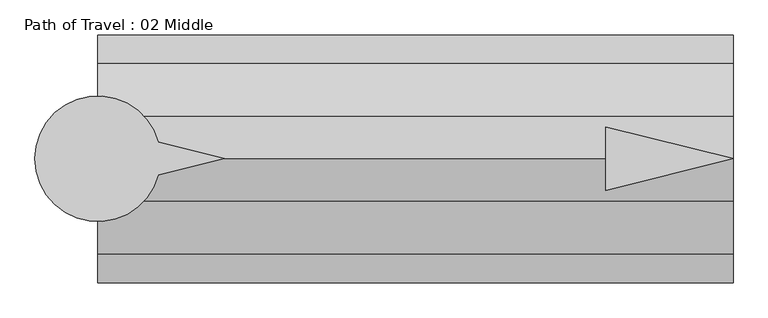
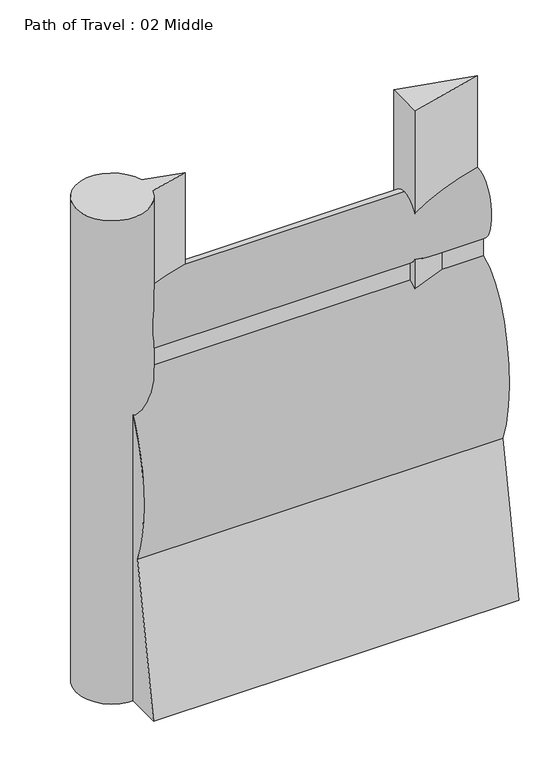
"""IFC4 building model written with IfcOpenShell, lengths in millimetres: proxy geometry, Path of Travel : 02 Middle."""

from ifc_helpers import new_model, si_unit, point, frame, frame_2d, origin, origin_with_axes, place, context, project, spatial, polyline, circle_curve, ellipse_curve, trimmed, segment, composite_curve, outline, extrude, source, transform, mapped, element, save
from ifc_brep_helpers import plane_surface, extruded_surface, advanced_brep


def path_of_travel_02_middle_987670bd(model_context):
    return source(origin(), model_context, "Body", "SolidModel", [
        advanced_brep(
        [(227.5554837, 0.0, 1727.2), (227.5554837, 42.9018657, 1436.6534209), (227.5554837, 42.9018657, 1363.4763406), (227.5554837, 184.1186263, 643.4144547), (227.5554837, 297.5699544, 0.0), (227.5554837, 145.6574193, 0.0), (227.5554837, 0.0, 584.2), (227.5554837, -145.6574193, 0.0), (227.5554837, -297.5699544, 0.0), (227.5554837, -184.1186263, 643.4144547), (227.5554837, -42.9018657, 1363.4763406), (227.5554837, -42.9018657, 1436.6534209), (1751.5554837, 0.0, 1727.2), (1751.5554837, -42.9018657, 1436.6534209), (1751.5554837, -42.9018657, 1363.4763406), (1751.5554837, -184.1186263, 643.4144547), (1751.5554837, -297.5699544, 0.0), (1751.5554837, -145.6574193, 0.0), (1751.5554837, 0.0, 584.2), (1751.5554837, 145.6574193, 0.0), (1751.5554837, 297.5699544, 0.0), (1751.5554837, 184.1186263, 643.4144547), (1751.5554837, 42.9018657, 1363.4763406), (1751.5554837, 42.9018657, 1436.6534209)],
        [
            (0, 1, ellipse_curve(frame((227.5554837, 0.0, 1574.8), z_axis=(-1.0, 0.0, 0.0), x_axis=(0.0, 0.0, 1.0)), 152.4, 101.6)),
            (1, 2),
            (2, 3, ellipse_curve(frame((227.5554837, 0.0, 914.4), z_axis=(-1.0, 0.0, 0.0), x_axis=(0.0, 0.0, -1.0)), 457.2, 228.6)),
            (3, 4),
            (4, 5),
            (5, 6),
            (6, 7),
            (7, 8),
            (8, 9),
            (9, 10, ellipse_curve(frame((227.5554837, 0.0, 914.4), z_axis=(-1.0, 0.0, 0.0), x_axis=(0.0, 0.0, -1.0)), 457.2, 228.6)),
            (10, 11),
            (11, 0, ellipse_curve(frame((227.5554837, 0.0, 1574.8), z_axis=(-1.0, 0.0, 0.0), x_axis=(0.0, 0.0, 1.0)), 152.4, 101.6)),
            (12, 13, ellipse_curve(frame((1751.5554837, 0.0, 1574.8), z_axis=(1.0, 0.0, 0.0), x_axis=(0.0, 0.0, 1.0)), 152.4, 101.6)),
            (13, 14),
            (14, 15, ellipse_curve(frame((1751.5554837, 0.0, 914.4), z_axis=(1.0, 0.0, 0.0), x_axis=(0.0, 0.0, -1.0)), 457.2, 228.6)),
            (15, 16),
            (16, 17),
            (17, 18),
            (18, 19),
            (19, 20),
            (20, 21),
            (21, 22, ellipse_curve(frame((1751.5554837, 0.0, 914.4), z_axis=(1.0, 0.0, 0.0), x_axis=(0.0, 0.0, -1.0)), 457.2, 228.6)),
            (22, 23),
            (23, 12, ellipse_curve(frame((1751.5554837, 0.0, 1574.8), z_axis=(1.0, 0.0, 0.0), x_axis=(0.0, 0.0, 1.0)), 152.4, 101.6)),
            (0, 12),
            (23, 1),
            (22, 2),
            (21, 3),
            (20, 4),
            (19, 5),
            (18, 6),
            (17, 7),
            (16, 8),
            (15, 9),
            (14, 10),
            (13, 11),
        ],
        [
            plane_surface(frame((227.5554837, 0.0, 0.0), z_axis=(-1.0, 0.0, 0.0), x_axis=(0.0, 0.0, 1.0))),
            plane_surface(frame((1751.5554837, 0.0, 0.0), z_axis=(1.0, 0.0, 0.0), x_axis=(0.0, 0.0, 1.0))),
            extruded_surface(trimmed(ellipse_curve(frame((1751.5554837, 0.0, 1574.8), z_axis=(-1.0, 0.0, 0.0), x_axis=(0.0, 0.0, 1.0)), 152.4, 101.6), [point((1751.5554837, 0.0, 1727.2))], [point((1751.5554837, 42.9018657, 1436.6534209))], True, "CARTESIAN"), (-1524.0, 0.0, 0.0), 1524.0),
            plane_surface(frame((227.5554837, 42.9018657, 1436.6534209), z_axis=(0.0, 1.0, 0.0), x_axis=(1.0, 0.0, 0.0))),
            extruded_surface(trimmed(ellipse_curve(frame((1751.5554837, 0.0, 914.4), z_axis=(-1.0, 0.0, 0.0), x_axis=(0.0, 0.0, -1.0)), 457.2, 228.6), [point((1751.5554837, 42.9018657, 1363.4763406))], [point((1751.5554837, 184.1186263, 643.4144547))], True, "CARTESIAN"), (-1524.0, 0.0, 0.0), 1524.0),
            plane_surface(frame((227.5554837, 184.1186263, 643.4144547), z_axis=(0.0, 0.9848077530122078, 0.1736481776669322), x_axis=(1.0, 0.0, 0.0))),
            plane_surface(frame((227.5554837, 297.5699544, 0.0), z_axis=(0.0, 0.0, -1.0), x_axis=(1.0, 0.0, 0.0))),
            plane_surface(frame((227.5554837, 145.6574193, 0.0), z_axis=(0.0, -0.9702957262760199, -0.2419218955995739), x_axis=(1.0, 0.0, 0.0))),
            plane_surface(frame((227.5554837, 0.0, 584.2), z_axis=(0.0, 0.9702957262759961, -0.24192189559966923), x_axis=(1.0, 0.0, 0.0))),
            plane_surface(frame((227.5554837, -145.6574193, 0.0), z_axis=(0.0, 0.0, -1.0), x_axis=(1.0, 0.0, 0.0))),
            plane_surface(frame((227.5554837, -297.5699544, 0.0), z_axis=(0.0, -0.984807753012208, 0.17364817766693066), x_axis=(1.0, 0.0, 0.0))),
            extruded_surface(trimmed(ellipse_curve(frame((1751.5554837, 0.0, 914.4), z_axis=(-1.0, 0.0, 0.0), x_axis=(0.0, 0.0, -1.0)), 457.2, 228.6), [point((1751.5554837, -184.1186263, 643.4144547))], [point((1751.5554837, -42.9018657, 1363.4763406))], True, "CARTESIAN"), (-1524.0, 0.0, 0.0), 1524.0),
            plane_surface(frame((227.5554837, -42.9018657, 1363.4763406), z_axis=(0.0, -1.0, 0.0), x_axis=(1.0, 0.0, 0.0))),
            extruded_surface(trimmed(ellipse_curve(frame((1751.5554837, 0.0, 1574.8), z_axis=(-1.0, 0.0, 0.0), x_axis=(0.0, 0.0, 1.0)), 152.4, 101.6), [point((1751.5554837, -42.9018657, 1436.6534209))], [point((1751.5554837, 0.0, 1727.2))], True, "CARTESIAN"), (-1524.0, 0.0, 0.0), 1524.0),
        ],
        [
            (0, [[1, 2, 3, 4, 5, 6, 7, 8, 9, 10, 11, 12]]),
            (1, [[13, 14, 15, 16, 17, 18, 19, 20, 21, 22, 23, 24]]),
            (2, [[-1, 25, -24, 26]]),
            (3, [[-2, -26, -23, 27]]),
            (4, [[-3, -27, -22, 28]]),
            (5, [[-4, -28, -21, 29]]),
            (6, [[-5, -29, -20, 30]]),
            (7, [[-6, -30, -19, 31]]),
            (8, [[-7, -31, -18, 32]]),
            (9, [[-8, -32, -17, 33]]),
            (10, [[-9, -33, -16, 34]]),
            (11, [[-10, -34, -15, 35]]),
            (12, [[-11, -35, -14, 36]]),
            (13, [[-12, -36, -13, -25]]),
        ],
    ),
        extrude(outline(polyline([(1445.5503371, 76.2006338), (1751.5554837, 0.0), (1445.5503371, -76.2006338), (1445.5503371, 76.2006338)])), origin_with_axes(), (0.0, 0.0, 1.0), 2129.5973753),
        extrude(outline(composite_curve([segment(polyline([(372.7837828, 39.4440225), (531.182385, 0.0), (372.7837828, -39.4440225)]), True, "CONTINUOUS"), segment(trimmed(circle_curve(frame_2d((227.2200886, 0.0)), 150.8131956), [point((372.7837828, -39.4440225))], [point((372.7837828, 39.4440225))], False, "CARTESIAN"), True, "CONTINUOUS")], self_intersect=False)), origin_with_axes(), (0.0, 0.0, 1.0), 2129.5973753),
    ])


if __name__ == "__main__":
    model = new_model("IFC4")
    model_context = context("Model", 3, world=origin())
    ifc_project = project(units=[si_unit("LENGTHUNIT", "METRE", prefix="MILLI")], contexts=[model_context])
    site = spatial("IfcSite", under=ifc_project)
    building = spatial("IfcBuilding", under=site)
    placement = place(None, origin())
    path_of_travel_02_middle_shape = path_of_travel_02_middle_987670bd(model_context)
    element("IfcBuildingElementProxy", 1, Name="Path of Travel : 02 Middle", ObjectType="Path of Travel : 02 Middle", at=placement, inside=building, context=model_context, shape_type="MappedRepresentation", body=[
        mapped(path_of_travel_02_middle_shape, transform((0.0, 0.0, 0.0), x_axis=(1.0, 0.0, 0.0), y_axis=(0.0, 1.0, 0.0), z_axis=(0.0, 0.0, 1.0))),
    ])
    save(model, "model.ifc")

# Revit data of these elements
# Type "Path of Travel : 02 Middle"
#   Path of Egress [instance default] = 4' - 0"
#   built-in parameter 1001306 [instance default] = 4 (stored number, unit not read)
#   Dot at Start = no
#   Arrow in Middle = yes
#   Arrow at End = no
#   Egress Path = none
# Element 1 (IfcBuildingElementProxy, "Path of Travel : 02 Middle")
#   Path of Egress = 5' - 0"
#   built-in parameter 1001306 = 5 (stored number, unit not read)
#   Materials on its faces: "Egress Path Solid", "solid"
# Materials
#   "Egress Path Solid": class "Unassigned", colour RGB 255 128 64, transparency 0.75, Comments = "Rendering appearance not upgraded "
#   "solid": class "Generic", colour RGB 120 120 120, transparency 0, Cost = 0
